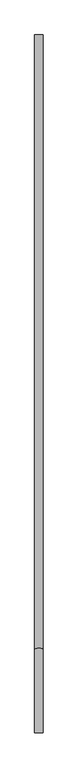
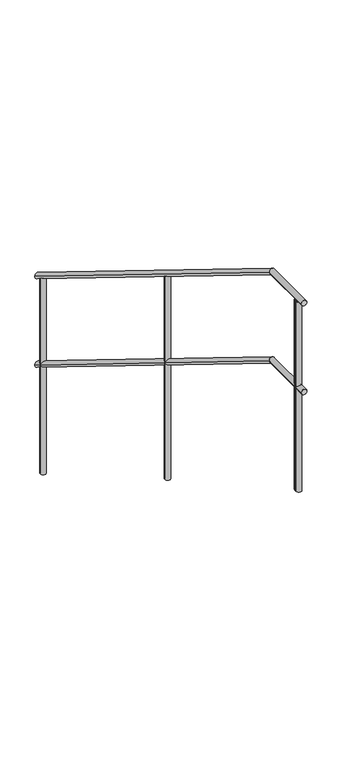
"""IFC4 building model written with IfcOpenShell, lengths in millimetres: railing geometry."""

from ifc_helpers import new_model, si_unit, point, frame, frame_2d, origin, place, context, project, spatial, circle_curve, ellipse_curve, trimmed, segment, composite_curve, outline, extrude, source, transform, mapped, element, save
from ifc_brep_helpers import plane_surface, cylinder_surface, advanced_brep


def railing_688346c1(model_context):
    return source(origin(), model_context, "Body", "SolidModel", [
        advanced_brep(
        [(-1026.0, 35476.2934796, -450.9609787), (-1056.0, 35476.2934796, -450.9609787), (-1056.0, 33312.0366941, 885.0), (-1026.0, 33312.0366941, 885.0), (-1026.0, 33016.2934796, 885.0), (-1056.0, 33016.2934796, 885.0)],
        [
            (0, 1, ellipse_curve(frame((-1041.0, 35476.2934796, -450.9609787), z_axis=(0.0, 1.0, 0.0), x_axis=(0.0, 0.0, -1.0)), 17.6276454, 15.0)),
            (1, 0, ellipse_curve(frame((-1041.0, 35476.2934796, -450.9609787), z_axis=(0.0, 1.0, 0.0), x_axis=(0.0, 0.0, -1.0)), 17.6276454, 15.0)),
            (1, 2),
            (2, 3, ellipse_curve(frame((-1041.0, 33312.0366941, 885.0), z_axis=(0.0, 0.9620125025549408, -0.2730053935877093), x_axis=(0.0, -0.27300539358770903, -0.962012502554941)), 15.5923129, 15.0)),
            (3, 0),
            (3, 2, ellipse_curve(frame((-1041.0, 33312.0366941, 885.0), z_axis=(0.0, 0.9620125025549408, -0.2730053935877093), x_axis=(0.0, -0.27300539358770903, -0.962012502554941)), 15.5923129, 15.0)),
            (4, 5, circle_curve(frame((-1041.0, 33016.2934796, 885.0), z_axis=(0.0, -1.0, 0.0), x_axis=(-1.0, 0.0, 0.0)), 15.0)),
            (5, 4, circle_curve(frame((-1041.0, 33016.2934796, 885.0), z_axis=(0.0, -1.0, 0.0), x_axis=(-1.0, 0.0, 0.0)), 15.0)),
            (2, 5),
            (4, 3),
        ],
        [
            plane_surface(frame((-1041.0, 35476.2934796, -433.3333333), z_axis=(0.0, 1.0, 0.0), x_axis=(0.0, 0.0, -1.0))),
            cylinder_surface(frame((-1041.0, 35468.4144415, -446.097375), z_axis=(0.0, 0.8509361101440399, -0.5252692037926177), x_axis=(-1.0, 0.0, 0.0)), 15.0),
            plane_surface(frame((-1041.0, 33016.2934796, 900.0), z_axis=(0.0, -1.0, 0.0), x_axis=(0.0, 0.0, -1.0))),
            cylinder_surface(frame((-1041.0, 33316.2934796, 885.0), z_axis=(0.0, 1.0, 0.0), x_axis=(-1.0, 0.0, 0.0)), 15.0),
        ],
        [
            (0, [[1, 2]]),
            (1, [[-2, 3, 4, 5]]),
            (1, [[-1, -5, 6, -3]]),
            (2, [[7, 8]]),
            (3, [[-4, 9, -7, 10]]),
            (3, [[-6, -10, -8, -9]]),
        ],
    ),
        advanced_brep(
        [(-1026.0, 35476.2934796, 49.0390213), (-1056.0, 35476.2934796, 49.0390213), (-1056.0, 33312.0366941, 1385.0), (-1026.0, 33312.0366941, 1385.0), (-1026.0, 33016.2934796, 1385.0), (-1056.0, 33016.2934796, 1385.0)],
        [
            (0, 1, ellipse_curve(frame((-1041.0, 35476.2934796, 49.0390213), z_axis=(0.0, 1.0, 0.0), x_axis=(0.0, 0.0, -1.0)), 17.6276454, 15.0)),
            (1, 0, ellipse_curve(frame((-1041.0, 35476.2934796, 49.0390213), z_axis=(0.0, 1.0, 0.0), x_axis=(0.0, 0.0, -1.0)), 17.6276454, 15.0)),
            (1, 2),
            (2, 3, ellipse_curve(frame((-1041.0, 33312.0366941, 1385.0), z_axis=(0.0, 0.9620125025549408, -0.2730053935877093), x_axis=(0.0, -0.27300539358770903, -0.962012502554941)), 15.5923129, 15.0)),
            (3, 0),
            (3, 2, ellipse_curve(frame((-1041.0, 33312.0366941, 1385.0), z_axis=(0.0, 0.9620125025549408, -0.2730053935877093), x_axis=(0.0, -0.27300539358770903, -0.962012502554941)), 15.5923129, 15.0)),
            (4, 5, circle_curve(frame((-1041.0, 33016.2934796, 1385.0), z_axis=(0.0, -1.0, 0.0), x_axis=(-1.0, 0.0, 0.0)), 15.0)),
            (5, 4, circle_curve(frame((-1041.0, 33016.2934796, 1385.0), z_axis=(0.0, -1.0, 0.0), x_axis=(-1.0, 0.0, 0.0)), 15.0)),
            (2, 5),
            (4, 3),
        ],
        [
            plane_surface(frame((-1041.0, 35476.2934796, 66.6666667), z_axis=(0.0, 1.0, 0.0), x_axis=(0.0, 0.0, -1.0))),
            cylinder_surface(frame((-1041.0, 35468.4144415, 53.902625), z_axis=(0.0, 0.8509361101440399, -0.5252692037926177), x_axis=(-1.0, 0.0, 0.0)), 15.0),
            plane_surface(frame((-1041.0, 33016.2934796, 1400.0), z_axis=(0.0, -1.0, 0.0), x_axis=(0.0, 0.0, -1.0))),
            cylinder_surface(frame((-1041.0, 33316.2934796, 1385.0), z_axis=(0.0, 1.0, 0.0), x_axis=(-1.0, 0.0, 0.0)), 15.0),
        ],
        [
            (0, [[1, 2]]),
            (1, [[-2, 3, 4, 5]]),
            (1, [[-1, -5, 6, -3]]),
            (2, [[7, 8]]),
            (3, [[-4, 9, -7, 10]]),
            (3, [[-6, -10, -8, -9]]),
        ],
    ),
        extrude(outline(composite_curve([segment(trimmed(circle_curve(frame_2d((-1041.0, 33076.2934796)), 15.0), [point((-1026.0, 33076.2934796))], [point((-1056.0, 33076.2934796))], False, "CARTESIAN"), True, "CONTINUOUS"), segment(trimmed(circle_curve(frame_2d((-1041.0, 33076.2934796)), 15.0), [point((-1056.0, 33076.2934796))], [point((-1026.0, 33076.2934796))], False, "CARTESIAN"), True, "CONTINUOUS")], self_intersect=False)), frame((0.0, 0.0, 300.0), z_axis=(0.0, 0.0, 1.0), x_axis=(1.0, 0.0, 0.0)), (0.0, 0.0, 1.0), 1070.0),
        advanced_brep(
        [(-1056.0, 34276.2934796, 777.4074074), (-1056.0, 34276.2934796, -366.6666667), (-1026.0, 34276.2934796, -366.6666667), (-1026.0, 34276.2934796, 777.4074074)],
        [
            (0, 1),
            (1, 2, circle_curve(frame((-1041.0, 34276.2934796, -366.6666667), z_axis=(0.0, 0.0, 1.0), x_axis=(1.0, 0.0, 0.0)), 15.0)),
            (2, 3),
            (3, 0, ellipse_curve(frame((-1041.0, 34276.2934796, 777.4074074), z_axis=(0.0, -0.5252692037926167, -0.8509361101440406), x_axis=(0.0, -0.8509361101440406, 0.5252692037926162)), 17.6276454, 15.0)),
            (0, 3, ellipse_curve(frame((-1041.0, 34276.2934796, 777.4074074), z_axis=(0.0, -0.5252692037926167, -0.8509361101440406), x_axis=(0.0, -0.8509361101440406, 0.5252692037926162)), 17.6276454, 15.0)),
            (2, 1, circle_curve(frame((-1041.0, 34276.2934796, -366.6666667), z_axis=(0.0, 0.0, 1.0), x_axis=(1.0, 0.0, 0.0)), 15.0)),
        ],
        [
            cylinder_surface(frame((-1041.0, 34276.2934796, -466.6666667), z_axis=(0.0, 0.0, 1.0), x_axis=(1.0, 0.0, 0.0)), 15.0),
            plane_surface(frame((-1016.0, 34251.2934796, 792.8395062), z_axis=(0.0, 0.5252692037926167, 0.8509361101440406), x_axis=(-1.0, 0.0, 0.0))),
            plane_surface(frame((-1016.0, 34301.2934796, -366.6666667), z_axis=(0.0, 0.0, -1.0), x_axis=(-1.0, 0.0, 0.0))),
        ],
        [
            (0, [[1, 2, 3, 4]]),
            (0, [[-1, 5, -3, 6]]),
            (1, [[-4, -5]]),
            (2, [[-2, -6]]),
        ],
    ),
        extrude(outline(composite_curve([segment(trimmed(circle_curve(frame_2d((-1041.0, 33066.2934796)), 15.0), [point((-1026.0, 33066.2934796))], [point((-1056.0, 33066.2934796))], False, "CARTESIAN"), True, "CONTINUOUS"), segment(trimmed(circle_curve(frame_2d((-1041.0, 33066.2934796)), 15.0), [point((-1056.0, 33066.2934796))], [point((-1026.0, 33066.2934796))], False, "CARTESIAN"), True, "CONTINUOUS")], self_intersect=False)), frame((0.0, 0.0, 300.0), z_axis=(0.0, 0.0, 1.0), x_axis=(1.0, 0.0, 0.0)), (0.0, 0.0, 1.0), 1070.0),
        advanced_brep(
        [(-1056.0, 35426.2934796, 67.5308642), (-1056.0, 35426.2934796, -1033.3333333), (-1026.0, 35426.2934796, -1033.3333333), (-1026.0, 35426.2934796, 67.5308642)],
        [
            (0, 1),
            (1, 2, circle_curve(frame((-1041.0, 35426.2934796, -1033.3333333), z_axis=(0.0, 0.0, 1.0), x_axis=(1.0, 0.0, 0.0)), 15.0)),
            (2, 3),
            (3, 0, ellipse_curve(frame((-1041.0, 35426.2934796, 67.5308642), z_axis=(0.0, -0.5252692037926167, -0.8509361101440406), x_axis=(0.0, -0.8509361101440406, 0.5252692037926162)), 17.6276454, 15.0)),
            (0, 3, ellipse_curve(frame((-1041.0, 35426.2934796, 67.5308642), z_axis=(0.0, -0.5252692037926167, -0.8509361101440406), x_axis=(0.0, -0.8509361101440406, 0.5252692037926162)), 17.6276454, 15.0)),
            (2, 1, circle_curve(frame((-1041.0, 35426.2934796, -1033.3333333), z_axis=(0.0, 0.0, 1.0), x_axis=(1.0, 0.0, 0.0)), 15.0)),
        ],
        [
            cylinder_surface(frame((-1041.0, 35426.2934796, -1133.3333333), z_axis=(0.0, 0.0, 1.0), x_axis=(1.0, 0.0, 0.0)), 15.0),
            plane_surface(frame((-1016.0, 35401.2934796, 82.962963), z_axis=(0.0, 0.5252692037926167, 0.8509361101440406), x_axis=(-1.0, 0.0, 0.0))),
            plane_surface(frame((-1016.0, 35451.2934796, -1033.3333333), z_axis=(0.0, 0.0, -1.0), x_axis=(-1.0, 0.0, 0.0))),
        ],
        [
            (0, [[1, 2, 3, 4]]),
            (0, [[-1, 5, -3, 6]]),
            (1, [[-4, -5]]),
            (2, [[-2, -6]]),
        ],
    ),
    ])


if __name__ == "__main__":
    model = new_model("IFC4")
    model_context = context("Model", 3, world=origin())
    ifc_project = project(units=[si_unit("LENGTHUNIT", "METRE", prefix="MILLI")], contexts=[model_context])
    site = spatial("IfcSite", under=ifc_project)
    building = spatial("IfcBuilding", under=site)
    placement = place(None, origin())
    railing_shape = railing_688346c1(model_context)
    element("IfcRailing", 1, at=placement, inside=building, context=model_context, shape_type="MappedRepresentation", body=[
        mapped(railing_shape, transform((0.0, 0.0, 0.0), x_axis=(1.0, 0.0, 0.0), y_axis=(0.0, 1.0, 0.0), z_axis=(0.0, 0.0, 1.0))),
    ])
    save(model, "model.ifc")
